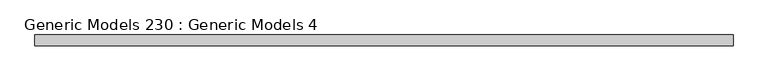
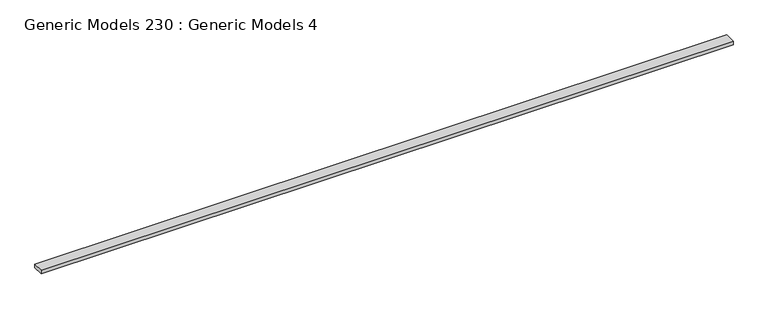
"""IFC4 building model written with IfcOpenShell, lengths in millimetres: proxy geometry, Generic Models 230 : Generic Models 4."""

from ifc_helpers import new_model, si_unit, frame, origin, place, context, project, spatial, polyline, outline, extrude, source, transform, mapped, element, save


def generic_models_230_generic_models_4_09111ff7(model_context):
    return source(origin(), model_context, "Body", "SweptSolid", [
        extrude(outline(polyline([(8409.0828684, 11786.1870839), (8409.0828684, 11499.2769662), (-10234.5171316, 11499.2769662), (-10234.5171316, 11786.1870839), (8409.0828684, 11786.1870839)])), frame((0.0, 0.0, 126821.946), z_axis=(0.0, 0.0, 1.0), x_axis=(1.0, 0.0, 0.0)), (0.0, 0.0, 1.0), 102.2351183),
    ])


if __name__ == "__main__":
    model = new_model("IFC4")
    model_context = context("Model", 3, world=origin())
    ifc_project = project(units=[si_unit("LENGTHUNIT", "METRE", prefix="MILLI")], contexts=[model_context])
    site = spatial("IfcSite", under=ifc_project)
    building = spatial("IfcBuilding", under=site)
    placement = place(None, origin())
    generic_models_230_generic_models_4_shape = generic_models_230_generic_models_4_09111ff7(model_context)
    element("IfcBuildingElementProxy", 1, Name="Generic Models 230 : Generic Models 4", ObjectType="Generic Models 230 : Generic Models 4", at=placement, inside=building, context=model_context, shape_type="MappedRepresentation", body=[
        mapped(generic_models_230_generic_models_4_shape, transform((0.0, 0.0, 0.0), x_axis=(1.0, 0.0, 0.0), y_axis=(0.0, 1.0, 0.0), z_axis=(0.0, 0.0, 1.0))),
    ])
    save(model, "model.ifc")

# Revit data of these elements
# Element 1 (IfcBuildingElementProxy, "Generic Models 230 : Generic Models 4")
#   Materials on its faces: "_TAPERED 2X BLOCKING (1% SLOPE) - SLOPED TOWARD DRAINS (SEE ROOF PLAN)"
# Materials
#   "_TAPERED 2X BLOCKING (1% SLOPE) - SLOPED TOWARD DRAINS (SEE ROOF PLAN)": class "Generic", colour RGB 177 130 114, transparency 0, Cost = 0
